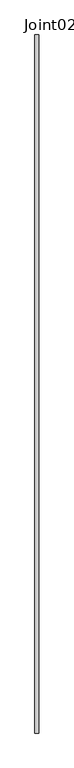
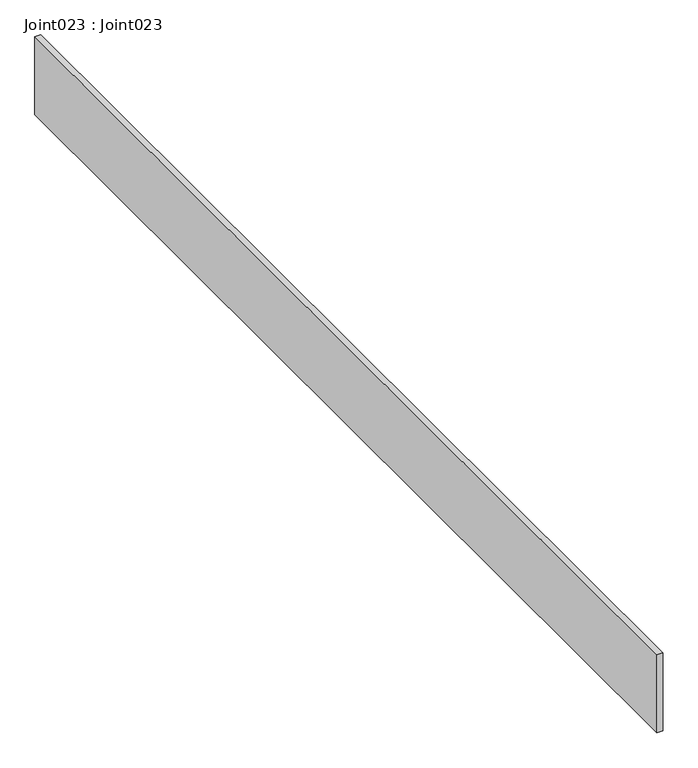
"""IFC4 building model written with IfcOpenShell, lengths in millimetres: proxy geometry, Joint023 : Joint023."""

from ifc_helpers import new_model, si_unit, frame, origin, place, context, project, spatial, polyline, outline, extrude, source, transform, mapped, element, save


def joint023_joint023_38171867(model_context):
    return source(origin(), model_context, "Body", "SweptSolid", [
        extrude(outline(polyline([(-10250.8737014, 7982.1531721), (-10261.8486328, 7982.1531721), (-10261.8486328, 9982.1531721), (-10250.8737014, 9982.1531721), (-10250.8737014, 7982.1531721)])), frame((0.0, 0.0, 32467.3000667), z_axis=(0.0, 0.0, 1.0), x_axis=(1.0, 0.0, 0.0)), (0.0, 0.0, 1.0), 152.4039393),
    ])


if __name__ == "__main__":
    model = new_model("IFC4")
    model_context = context("Model", 3, world=origin())
    ifc_project = project(units=[si_unit("LENGTHUNIT", "METRE", prefix="MILLI")], contexts=[model_context])
    site = spatial("IfcSite", under=ifc_project)
    building = spatial("IfcBuilding", under=site)
    placement = place(None, origin())
    joint023_joint023_shape = joint023_joint023_38171867(model_context)
    element("IfcBuildingElementProxy", 1, Name="Joint023 : Joint023", ObjectType="Joint023 : Joint023", at=placement, inside=building, context=model_context, shape_type="MappedRepresentation", body=[
        mapped(joint023_joint023_shape, transform((0.0, 0.0, 0.0), x_axis=(1.0, 0.0, 0.0), y_axis=(0.0, 1.0, 0.0), z_axis=(0.0, 0.0, 1.0))),
    ])
    save(model, "model.ifc")

# Revit data of these elements
# Type "Joint023 : Joint023"
#   NameOverride = "Joint023"
# Element 1 (IfcBuildingElementProxy, "Joint023 : Joint023")
#   Materials on its faces: "CONCRETE EXPANSION JOINT - MINERAL FIBER"
# Materials
#   "CONCRETE EXPANSION JOINT - MINERAL FIBER": class "Unassigned", colour RGB 82 203 28, transparency 0
